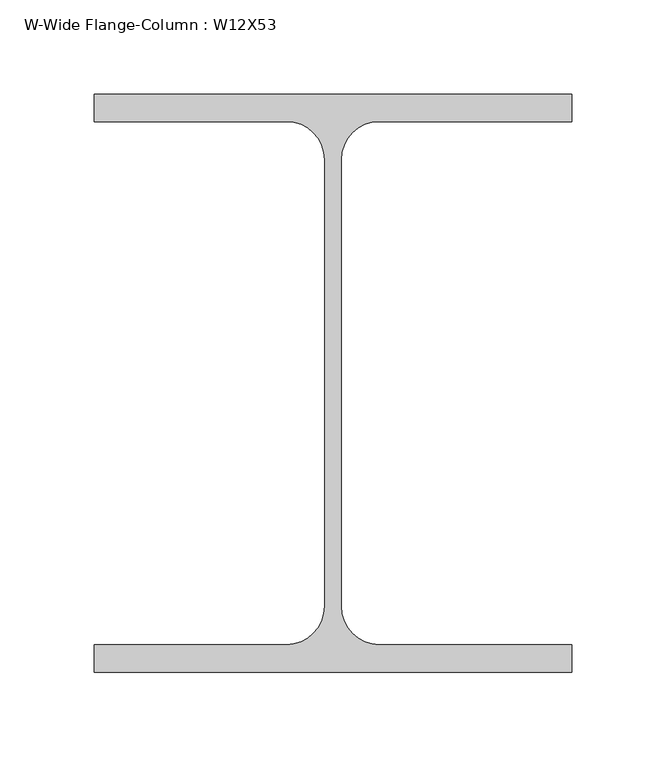
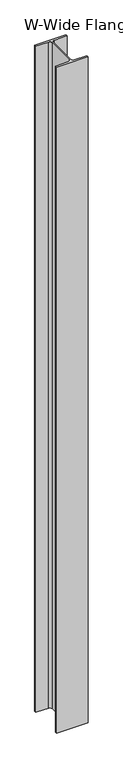
"""IFC4 building model written with IfcOpenShell, lengths in millimetres: column geometry, W-Wide Flange-Column : W12X53."""

import ifcopenshell
import ifcopenshell.guid

model = None  # the IFC model being written
_history = None  # IfcOwnerHistory: only IFC2X3 demands one
_inside = {}  # id of a spatial element -> (the spatial element, [elements in it])
_under = {}  # id of a project, library or spatial element -> (it, [spatial elements below it])
_declared = {}  # id of a project -> (the project, [libraries it declares])
_typed = {}  # id of a type object -> (the type object, [elements of that type])
_made_of = {}  # id of a material, layer set ... -> (it, [elements and type objects made of it])


def new_model(schema):
    """Start an empty IFC model of exactly this schema.

    Asked for "IFC4X3", IfcOpenShell would pick the latest addendum, in which some entities
    have other attributes; the version numbers below select the first issue.
    IFC2X3 requires an IfcOwnerHistory on every rooted entity: one is made here for all.
    """
    global model, _history
    if schema == "IFC4X3":
        model = ifcopenshell.file(schema_version=(4, 3, 0, 0))
    else:
        model = ifcopenshell.file(schema=schema)
    _inside.clear()
    _under.clear()
    _declared.clear()
    _typed.clear()
    _made_of.clear()
    _history = None
    if model.schema == "IFC2X3":
        org = make("IfcOrganization", Name="unknown")
        user = make(
            "IfcPersonAndOrganization",
            ThePerson=make("IfcPerson", FamilyName="unknown"),
            TheOrganization=org,
        )
        app = make(
            "IfcApplication",
            ApplicationDeveloper=org,
            Version="unknown",
            ApplicationFullName="unknown",
            ApplicationIdentifier="unknown",
        )
        _history = make(
            "IfcOwnerHistory",
            OwningUser=user,
            OwningApplication=app,
            ChangeAction="ADDED",
            CreationDate=0,
        )
    return model


def make(cls, **values):
    """One entity of the class cls with the attributes given. An attribute that is None is left unset."""
    return model.create_entity(
        cls, **{name: value for name, value in values.items() if value is not None}
    )


def rooted(cls, **values):
    """An entity with a GlobalId (a new one), such as an element, a storey or a relation."""
    return make(cls, GlobalId=ifcopenshell.guid.new(), OwnerHistory=_history, **values)


def si_unit(unit_type, name, prefix=None):
    """IfcSIUnit, for example si_unit("LENGTHUNIT", "METRE", prefix="MILLI")."""
    return make("IfcSIUnit", UnitType=unit_type, Prefix=prefix, Name=name)


def assignment(units):
    """IfcUnitAssignment: the units of a project."""
    return None if units is None else make("IfcUnitAssignment", Units=units)


def point(xyz):
    """IfcCartesianPoint."""
    return None if xyz is None else make("IfcCartesianPoint", Coordinates=xyz)


def direction(xyz):
    """IfcDirection."""
    return None if xyz is None else make("IfcDirection", DirectionRatios=xyz)


def frame(location, z_axis=None, x_axis=None):
    """IfcAxis2Placement3D, a coordinate frame: its origin and axes. An axis left out is left unset."""
    return make(
        "IfcAxis2Placement3D",
        Location=point(location),
        Axis=direction(z_axis),
        RefDirection=direction(x_axis),
    )


def frame_2d(location, x_axis=None):
    """IfcAxis2Placement2D, a coordinate frame in the plane: its origin and x axis."""
    return make(
        "IfcAxis2Placement2D", Location=point(location), RefDirection=direction(x_axis)
    )


def origin():
    """The frame at (0, 0, 0) with its axes left unset."""
    return frame((0.0, 0.0, 0.0))


def place(relative_to, where):
    """IfcLocalPlacement: puts the frame where relative to a parent placement (None: the world)."""
    return make(
        "IfcLocalPlacement", PlacementRelTo=relative_to, RelativePlacement=where
    )


def context(
    kind, dimensions, precision=None, world=None, true_north=None, identifier=None
):
    """IfcGeometricRepresentationContext, for example the 3D "Model" context."""
    return make(
        "IfcGeometricRepresentationContext",
        ContextIdentifier=identifier,
        ContextType=kind,
        CoordinateSpaceDimension=dimensions,
        Precision=precision,
        WorldCoordinateSystem=world,
        TrueNorth=true_north,
    )


def project(units=None, contexts=None):
    """IfcProject with its units and contexts."""
    return rooted(
        "IfcProject",
        Name="project",
        RepresentationContexts=contexts,
        UnitsInContext=assignment(units),
    )


def spatial(cls, under=None, at=None, **own):
    """A site, building, storey or space (cls), placed at a placement, below another one or the project."""
    s = rooted(cls, ObjectPlacement=at, **own)
    if under is not None:
        _under.setdefault(under.id(), (under, []))[1].append(s)
    return s


def polyline(points):
    """IfcPolyline through the points."""
    return make("IfcPolyline", Points=[point(p) for p in points])


def circle_curve(where, radius):
    """IfcCircle in the frame where."""
    return make("IfcCircle", Position=where, Radius=radius)


def trimmed(basis, trim1, trim2, sense, master):
    """IfcTrimmedCurve: the piece of a basis curve between two trims."""
    return make(
        "IfcTrimmedCurve",
        BasisCurve=basis,
        Trim1=trim1,
        Trim2=trim2,
        SenseAgreement=sense,
        MasterRepresentation=master,
    )


def segment(curve, same_sense, transition):
    """IfcCompositeCurveSegment."""
    return make(
        "IfcCompositeCurveSegment",
        Transition=transition,
        SameSense=same_sense,
        ParentCurve=curve,
    )


def composite_curve(segments, self_intersect=None):
    """IfcCompositeCurve: segments joined end to end."""
    return make("IfcCompositeCurve", Segments=segments, SelfIntersect=self_intersect)


def outline(outer, holes=None, kind="AREA"):
    """IfcArbitraryClosedProfileDef: a profile drawn as a closed curve; with holes, ...WithVoids."""
    if holes is None:
        return make("IfcArbitraryClosedProfileDef", ProfileType=kind, OuterCurve=outer)
    return make(
        "IfcArbitraryProfileDefWithVoids",
        ProfileType=kind,
        OuterCurve=outer,
        InnerCurves=holes,
    )


def extrude(swept, where, along, depth):
    """IfcExtrudedAreaSolid: the profile swept, set in the frame where, extruded along a direction by depth."""
    return make(
        "IfcExtrudedAreaSolid",
        SweptArea=swept,
        Position=where,
        ExtrudedDirection=direction(along),
        Depth=depth,
    )


def shape(context_of_items, identifier, shape_type, items):
    """IfcShapeRepresentation: the items that make up one representation, for example the "Body"."""
    return make(
        "IfcShapeRepresentation",
        ContextOfItems=context_of_items,
        RepresentationIdentifier=identifier,
        RepresentationType=shape_type,
        Items=items,
    )


def source(mapping_origin, context_of_items, identifier, shape_type, items):
    """IfcRepresentationMap: a shape defined once, which mapped items show again and again."""
    return make(
        "IfcRepresentationMap",
        MappingOrigin=mapping_origin,
        MappedRepresentation=shape(context_of_items, identifier, shape_type, items),
    )


def transform(
    local_origin,
    x_axis=None,
    y_axis=None,
    z_axis=None,
    scale=None,
    scale2=None,
    scale3=None,
    uniform=True,
):
    """IfcCartesianTransformationOperator3D, or its non-uniform kind. x_axis, y_axis, z_axis: its Axis1, 2, 3."""
    if uniform:
        return make(
            "IfcCartesianTransformationOperator3D",
            Axis1=direction(x_axis),
            Axis2=direction(y_axis),
            LocalOrigin=point(local_origin),
            Scale=scale,
            Axis3=direction(z_axis),
        )
    return make(
        "IfcCartesianTransformationOperator3DnonUniform",
        Axis1=direction(x_axis),
        Axis2=direction(y_axis),
        LocalOrigin=point(local_origin),
        Scale=scale,
        Axis3=direction(z_axis),
        Scale2=scale2,
        Scale3=scale3,
    )


def mapped(mapping_source, mapping_target):
    """IfcMappedItem: shows the shape of a source again, moved by a transform."""
    return make(
        "IfcMappedItem", MappingSource=mapping_source, MappingTarget=mapping_target
    )


def made_of(thing, what):
    """Note that an element or type object is made of a material, layer set ...; save() writes the relation."""
    if what is not None:
        _made_of.setdefault(what.id(), (what, []))[1].append(thing)
    return thing


def element(
    cls,
    number,
    at=None,
    inside=None,
    cuts=None,
    type_object=None,
    material=None,
    context=None,
    identifier="Body",
    shape_type=None,
    held_by="IfcProductDefinitionShape",
    body=None,
    shapes=None,
    **own,
):
    """One element of the class cls, such as IfcWall. Its Tag is "e" and its number.

    at: its placement. inside: the storey or other place that contains it. cuts: it is an
    opening in that element (IfcRelVoidsElement). A single representation is given by context,
    identifier, shape_type and body (its items); several are given by shapes. held_by: the class
    of the entity that holds the representations. save() writes the other relations.
    """
    e = rooted(cls, Tag="e%d" % number, ObjectPlacement=at, **own)
    if body is not None:
        shapes = [shape(context, identifier, shape_type, body)]
    if shapes is not None:
        e.Representation = make(held_by, Representations=shapes)
    if inside is not None:
        _inside.setdefault(inside.id(), (inside, []))[1].append(e)
    if cuts is not None:
        rooted(
            "IfcRelVoidsElement", RelatingBuildingElement=cuts, RelatedOpeningElement=e
        )
    if type_object is not None:
        _typed.setdefault(type_object.id(), (type_object, []))[1].append(e)
    return made_of(e, material)


def aggregate(whole, parts):
    """IfcRelAggregates: a whole, such as a stair, and the parts it consists of."""
    return rooted("IfcRelAggregates", RelatingObject=whole, RelatedObjects=parts)


def save(model, path):
    """Write the relations noted so far, then the file.

    IfcRelAggregates (storeys below a building ...), IfcRelContainedInSpatialStructure (elements
    in a storey), IfcRelDefinesByType, IfcRelAssociatesMaterial and IfcRelDeclares: one each for
    every whole, place, type object, material and project.
    """
    for whole, parts in _under.values():
        aggregate(whole, parts)
    for where, things in _inside.values():
        rooted(
            "IfcRelContainedInSpatialStructure",
            RelatedElements=things,
            RelatingStructure=where,
        )
    for kind, things in _typed.values():
        rooted("IfcRelDefinesByType", RelatedObjects=things, RelatingType=kind)
    for what, things in _made_of.values():
        rooted("IfcRelAssociatesMaterial", RelatedObjects=things, RelatingMaterial=what)
    for by, libraries in _declared.values():
        rooted("IfcRelDeclares", RelatingContext=by, RelatedDefinitions=libraries)
    model.write(path)


def w_wide_flange_column_w12x53_a2bdef27(model_context):
    return source(origin(), model_context, "Body", "SweptSolid", [
        extrude(outline(composite_curve([segment(polyline([(127.0, 153.67), (127.0, 139.065), (24.7015, 139.065)]), True, "CONTINUOUS"), segment(trimmed(circle_curve(frame_2d((24.7015, 118.745)), 20.32), [point((24.7015, 139.065))], [point((4.3815, 118.745))], True, "CARTESIAN"), True, "CONTINUOUS"), segment(polyline([(4.3815, 118.745), (4.3815, -118.745)]), True, "CONTINUOUS"), segment(trimmed(circle_curve(frame_2d((24.7015, -118.745)), 20.32), [point((4.3815, -118.745))], [point((24.7015, -139.065))], True, "CARTESIAN"), True, "CONTINUOUS"), segment(polyline([(24.7015, -139.065), (127.0, -139.065), (127.0, -153.67), (-127.0, -153.67), (-127.0, -139.065), (-24.7015, -139.065)]), True, "CONTINUOUS"), segment(trimmed(circle_curve(frame_2d((-24.7015, -118.745)), 20.32), [point((-24.7015, -139.065))], [point((-4.3815, -118.745))], True, "CARTESIAN"), True, "CONTINUOUS"), segment(polyline([(-4.3815, -118.745), (-4.3815, 118.745)]), True, "CONTINUOUS"), segment(trimmed(circle_curve(frame_2d((-24.7015, 118.745)), 20.32), [point((-4.3815, 118.745))], [point((-24.7015, 139.065))], True, "CARTESIAN"), True, "CONTINUOUS"), segment(polyline([(-24.7015, 139.065), (-127.0, 139.065), (-127.0, 153.67), (127.0, 153.67)]), True, "CONTINUOUS")], self_intersect=False)), frame((0.0, 0.0, 23317.2), z_axis=(0.0, 0.0, 1.0), x_axis=(1.0, 0.0, 0.0)), (0.0, 0.0, 1.0), 5689.6),
    ])


if __name__ == "__main__":
    model = new_model("IFC4")
    model_context = context("Model", 3, world=origin())
    ifc_project = project(units=[si_unit("LENGTHUNIT", "METRE", prefix="MILLI")], contexts=[model_context])
    site = spatial("IfcSite", under=ifc_project)
    building = spatial("IfcBuilding", under=site)
    placement = place(None, origin())
    w_wide_flange_column_w12x53_shape = w_wide_flange_column_w12x53_a2bdef27(model_context)
    element("IfcColumn", 1, ObjectType="W-Wide Flange-Column : W12X53", at=placement, inside=building, context=model_context, shape_type="MappedRepresentation", body=[
        mapped(w_wide_flange_column_w12x53_shape, transform((0.0, 0.0, 0.0), x_axis=(1.0, 0.0, 0.0), y_axis=(0.0, 1.0, 0.0), z_axis=(0.0, 0.0, 1.0))),
    ])
    save(model, "model.ifc")

# Revit data of these elements
# Type "W-Wide Flange-Column : W12X53"
#   Assembly Code = "B10"
#   W = 53
#   bf = 0' - 10"
#   d = 1' - 0.1"
#   k = 0' - 1 3/8"
#   kr = 0' - 0.8"
#   tf = 0' - 0.575"
#   tw = 0' - 0.345"
#   A = 0.108333 SF
#   Structural Material [instance default] = Steel ASTM A992
# Element 1 (IfcColumn, "W-Wide Flange-Column : W12X53")
#   Materials on its faces: "Steel ASTM A992"
# Materials
#   "Steel ASTM A992": class "Metal", colour RGB 199 199 199, transparency 0, Description = "Structural steel 50ksi", Cost = 0
